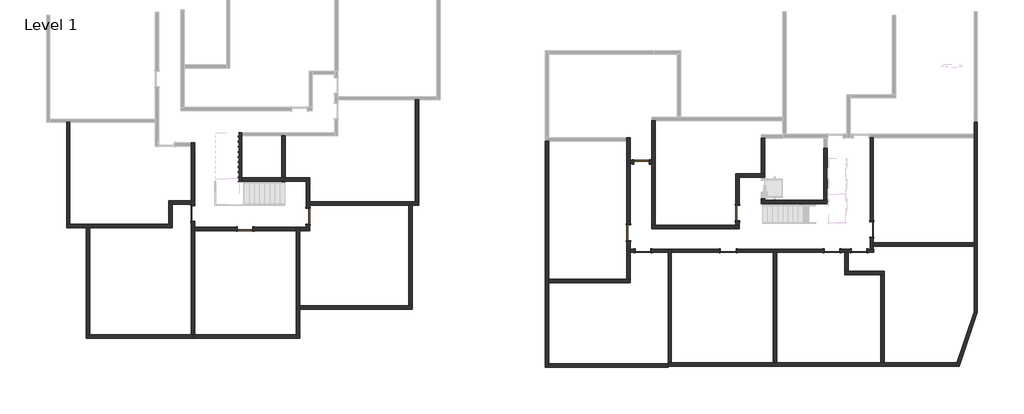
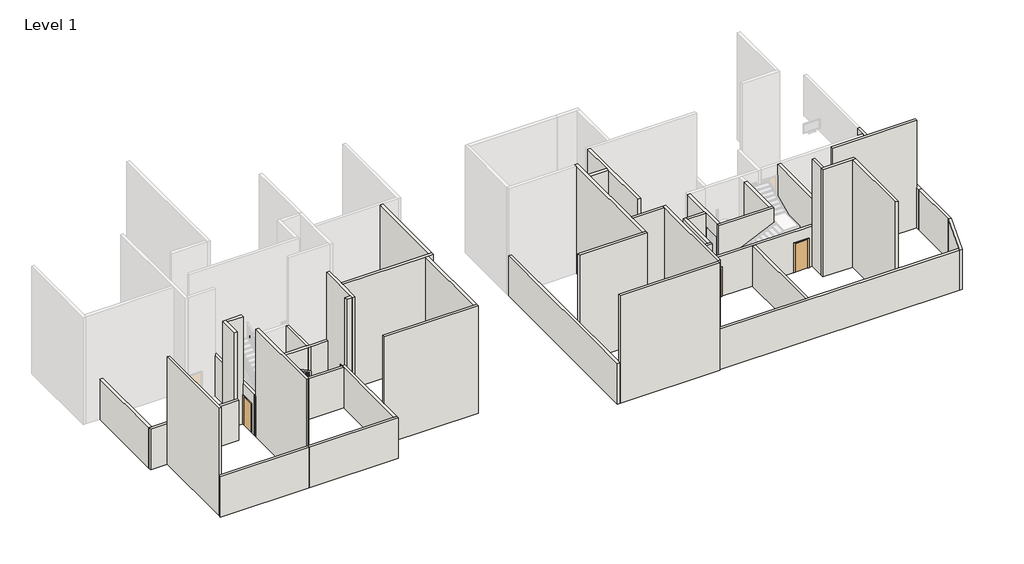
# One storey, part 1 of 3: 45 walls, 11 doors.
# Revit data of these elements (continued)
# Room at (24094.006, 1386.264) mm, phase "New Construction", upper level "Level 1", upper offset 243.84 cm, lower offset 0 cm (continued)
#   Name = "1"
# Room, not placed, phase "New Construction", upper offset 0 cm, lower offset 0 cm
#   Number = "81"
#   Name = "Room"
# Room, not placed, phase "New Construction", upper offset 0 cm, lower offset 0 cm
#   Number = "82"
#   Name = "Room"
# Room, not placed, phase "New Construction", upper offset 0 cm, lower offset 0 cm
#   Number = "83"
#   Name = "Room"
# Room, not placed, phase "New Construction", upper offset 0 cm, lower offset 0 cm
#   Number = "84"
#   Name = "5"
# Room, not placed, phase "New Construction", upper offset 0 cm, lower offset 0 cm
#   Number = "85"
#   Name = "Room"
# Room, not placed, phase "New Construction", upper offset 0 cm, lower offset 0 cm
#   Number = "18"
#   Name = "Room"
# Room, not placed, phase "New Construction", upper offset 0 cm, lower offset 0 cm
#   Number = "86"
#   Name = "Room"
# Room, not placed, phase "New Construction", upper offset 0 cm, lower offset 0 cm
#   Number = "137"
#   Name = "Room"
# Room at (15996.482, -9926.883) mm, phase "New Construction", upper level "Level 1", upper offset 243.84 cm, lower offset 0 cm
#   Number = "121"
#   Name = "5"
# Room at (9621.564, -11578.797) mm, phase "New Construction", upper level "Level 1", upper offset 243.84 cm, lower offset 0 cm
#   Number = "122"
#   Name = "6"
# Room at (20140.22, -1678.403) mm, phase "New Construction", upper level "Level 1", upper offset 243.84 cm, lower offset 0 cm
#   Number = ""
#   Name = "ASANSÖR"
# Room at (18694.214, -4908.781) mm, phase "New Construction", upper level "Level 1", upper offset 243.84 cm, lower offset 0 cm
#   Number = "49"
#   Name = "Room"
# Room, not placed, phase "New Construction", upper offset 0 cm, lower offset 0 cm
#   Number = "50"
#   Name = "Room"
# Room, not placed, phase "New Construction", upper offset 0 cm, lower offset 0 cm
#   Number = "51"
#   Name = "Room"
# Room, not placed, phase "New Construction", upper offset 0 cm, lower offset 0 cm
#   Number = "52"
#   Name = "Room"
# Room, not placed, phase "New Construction", upper offset 0 cm, lower offset 0 cm
#   Number = "53"
#   Name = "Room"
# Room, not placed, phase "New Construction", upper offset 0 cm, lower offset 0 cm
#   Number = "54"
#   Name = "Room"
# Room, not placed, phase "New Construction", upper offset 0 cm, lower offset 0 cm
#   Number = "55"
#   Name = "Room"
# Room, not placed, phase "New Construction", upper offset 0 cm, lower offset 0 cm
#   Number = "56"
#   Name = "Room"
# Room, not placed, phase "New Construction", upper offset 0 cm, lower offset 0 cm
#   Number = ""
#   Name = "Çamaşır- Kombi"
# Room, not placed, phase "New Construction", upper offset 0 cm, lower offset 0 cm
#   Number = "32"
#   Name = "Room"
# Room, not placed, phase "New Construction", upper offset 0 cm, lower offset 0 cm
#   Number = "33"
#   Name = "Room"
# Room at (7488.93, 2835.695) mm, phase "New Construction", upper level "Level 1", upper offset 243.84 cm, lower offset 0 cm
#   Number = "148"
#   Name = "8"
# Room at (7233.818, -6985.691) mm, phase "New Construction", upper level "Level 1", upper offset 243.84 cm, lower offset 0 cm
#   Number = "123"
#   Name = "7"
# Room, not placed, phase "New Construction", upper offset 0 cm, lower offset 0 cm
#   Number = "138"
#   Name = "Room"
# Room at (25542.506, -4072.569) mm, phase "New Construction", upper level "Level 1", upper offset 243.84 cm, lower offset 0 cm
#   Number = "87"
#   Name = "2"
# Room at (21725.305, -10013.945) mm, phase "New Construction", upper level "Level 1", upper offset 243.84 cm, lower offset 0 cm
#   Number = "88"
#   Name = "4"
# Area at (20046.111, 5871.007) mm, upper offset 243.84 cm, lower offset 0 cm
#   Number = "12"
#   Name = "Area"
# Room at (-4310.78, -978.519) mm, phase "New Construction", upper level "Level 1", upper offset 243.84 cm, lower offset 0 cm
#   Number = "149"
#   Name = "7"
# Room, not placed, phase "New Construction", upper offset 0 cm, lower offset 0 cm
#   Number = "57"
#   Name = "Room"
# Room, not placed, phase "New Construction", upper offset 0 cm, lower offset 0 cm
#   Number = ""
#   Name = "Room"
# Room, not placed, phase "New Construction", upper offset 0 cm, lower offset 0 cm
#   Number = "59"
#   Name = "Room"
# Room, not placed, phase "New Construction", upper offset 0 cm, lower offset 0 cm
#   Number = "60"
#   Name = "Room"
# Room, not placed, phase "New Construction", upper offset 0 cm, lower offset 0 cm
#   Number = "61"
#   Name = "Room"
# Room, not placed, phase "New Construction", upper offset 0 cm, lower offset 0 cm
#   Number = "62"
#   Name = "Room"
# Room, not placed, phase "New Construction", upper offset 0 cm, lower offset 0 cm
#   Number = "63"
#   Name = "Room"
# Area, not placed, upper offset 0 cm, lower offset 0 cm
#   Number = "5"
#   Name = "Dere Parsel Toplam Alan"
# Room, not placed, phase "New Construction", upper offset 0 cm, lower offset 0 cm
#   Number = "67"
#   Name = "Room"
# Room, not placed, phase "New Construction", upper offset 0 cm, lower offset 0 cm
#   Number = "68"
#   Name = "Room"
# Room at (-14817.024, 11588.139) mm, phase "New Construction", upper level "Level 1", upper offset 243.84 cm, lower offset 0 cm
#   Number = "139"
#   Name = "10"
# Room at (27717.749, -8269.379) mm, phase "New Construction", upper level "Level 1", upper offset 243.84 cm, lower offset 0 cm
#   Number = "90"
#   Name = "3"
# Area, not placed, upper offset 0 cm, lower offset 0 cm
#   Number = "6"
#   Name = "Area"
# Room, not placed, phase "New Construction", upper offset 0 cm, lower offset 0 cm
#   Number = "93"
#   Name = "6"
# Room, not placed, phase "New Construction", upper offset 0 cm, lower offset 0 cm
#   Number = "5"
#   Name = "Room"
# Room, not placed, phase "New Construction", upper offset 0 cm, lower offset 0 cm
#   Number = "6"
#   Name = "Room"
# Room, not placed, phase "New Construction", upper offset 0 cm, lower offset 0 cm
#   Number = "124"
#   Name = "Room"
# Room at (-20992.701, 5104.389) mm, phase "New Construction", upper level "Level 1", upper offset 243.84 cm, lower offset 0 cm
#   Number = "140"
#   Name = "2"
# Room at (-18388.177, -3094.154) mm, phase "New Construction", upper level "Level 1", upper offset 243.84 cm, lower offset 0 cm
#   Number = "141"
#   Name = "3"
# Room, not placed, phase "New Construction", upper offset 0 cm, lower offset 0 cm
#   Number = "34"
#   Name = "Room"
# Room, not placed, phase "New Construction", upper offset 0 cm, lower offset 0 cm
#   Number = "35"
#   Name = "Room"
# Room, not placed, phase "New Construction", upper offset 0 cm, lower offset 0 cm
#   Number = "9"
#   Name = "Room"
# Room, not placed, phase "New Construction", upper offset 0 cm, lower offset 0 cm
#   Number = "10"
#   Name = "Room"
# Room, not placed, phase "New Construction", upper offset 0 cm, lower offset 0 cm
#   Number = "125"
#   Name = "Room"
# Room, not placed, phase "New Construction", upper offset 0 cm, lower offset 0 cm
#   Number = "126"
#   Name = "Room"
# Room, not placed, phase "New Construction", upper offset 0 cm, lower offset 0 cm
#   Number = "127"
#   Name = "Room"
# Room, not placed, phase "New Construction", upper offset 0 cm, lower offset 0 cm
#   Number = "128"
#   Name = "Room"
# Room, not placed, phase "New Construction", upper offset 0 cm, lower offset 0 cm
#   Number = "129"
#   Name = "Room"
# Room, not placed, phase "New Construction", upper offset 0 cm, lower offset 0 cm
#   Number = "91"
#   Name = "Room"
# Room at (-21021.225, 8802.195) mm, phase "New Construction", upper level "Level 1", upper offset 243.84 cm, lower offset 0 cm
#   Number = "130"
#   Name = "1"
# Room at (-7083.952, -9470.79) mm, phase "New Construction", upper level "Level 1", upper offset 243.84 cm, lower offset 0 cm
#   Number = "131"
#   Name = "6"
# Room, not placed, phase "New Construction", upper offset 0 cm, lower offset 0 cm
#   Number = "132"
#   Name = "Room"
# Room, not placed, phase "New Construction", upper offset 0 cm, lower offset 0 cm
#   Number = "133"
#   Name = "Room"
# Room, not placed, phase "New Construction", upper offset 0 cm, lower offset 0 cm
#   Number = ""
#   Name = ""
# Room, not placed, phase "New Construction", upper offset 0 cm, lower offset 0 cm
#   Number = "70"
#   Name = "Room"
# Room, not placed, phase "New Construction", upper offset 0 cm, lower offset 0 cm
#   Number = "71"
#   Name = "Room"
# Room at (-18795.413, -7606.788) mm, phase "New Construction", upper level "Level 1", upper offset 243.84 cm, lower offset 0 cm
#   Number = "150"
#   Name = "4"
# Room at (43355.762, -8638.307) mm, phase "New Construction", upper level "Level 1", upper offset 243.84 cm, lower offset 0 cm
#   Number = "151"
#   Name = "Room"
# Room, not placed, phase "New Construction", upper offset 0 cm, lower offset 0 cm
#   Number = "92"
#   Name = "Room"
# Room, not placed, phase "New Construction", upper offset 0 cm, lower offset 0 cm
#   Number = ""
#   Name = ""
# Area, not placed, upper offset 0 cm, lower offset 0 cm
#   Number = "10"
#   Name = "Area"
# Area, not placed, upper offset 0 cm, lower offset 0 cm
#   Number = "11"
#   Name = "Area"
# Room, not placed, phase "New Construction", upper offset 0 cm, lower offset 0 cm
#   Number = ""
#   Name = ""
# Room, not placed, phase "New Construction", upper offset 0 cm, lower offset 0 cm
#   Number = "37"
#   Name = "Room"
# Room, not placed, phase "New Construction", upper offset 0 cm, lower offset 0 cm
#   Number = ""
#   Name = "Banyo"
# Room, not placed, phase "New Construction", upper offset 0 cm, lower offset 0 cm
#   Number = ""
#   Name = ""
# Room, not placed, phase "New Construction", upper offset 0 cm, lower offset 0 cm
#   Number = ""
#   Name = "Yatak Odası"
# Room, not placed, phase "New Construction", upper offset 0 cm, lower offset 0 cm
#   Number = "39"
#   Name = "Room"
# Room, not placed, phase "New Construction", upper offset 0 cm, lower offset 0 cm
#   Number = ""
#   Name = "Salon-Mutfak"
# Area, not placed, upper offset 0 cm, lower offset 0 cm
#   Number = "9"
#   Name = "Area"
# Room, not placed, phase "New Construction", upper offset 0 cm, lower offset 0 cm
#   Number = "134"
#   Name = "Room"
# Room, not placed, phase "New Construction", upper offset 0 cm, lower offset 0 cm
#   Number = "135"
#   Name = "Room"
# Room, not placed, phase "New Construction", upper offset 0 cm, lower offset 0 cm
#   Number = "40"
#   Name = "Room"
# Room, not placed, phase "New Construction", upper offset 0 cm, lower offset 0 cm
#   Number = "41"
#   Name = "Room"
# Room at (-12703.035, -7311.307) mm, phase "New Construction", upper level "Level 1", upper offset 243.84 cm, lower offset 0 cm
#   Number = "142"
#   Name = "5"
# Room, not placed, phase "New Construction", upper offset 0 cm, lower offset 0 cm
#   Number = "143"
#   Name = "Room"
# Room, not placed, phase "New Construction", upper offset 0 cm, lower offset 0 cm
#   Number = "144"
#   Name = "Room"
# Room at (-12608.918, 6644.855) mm, phase "New Construction", upper level "Level 1", upper offset 243.84 cm, lower offset 0 cm
#   Number = "145"
#   Name = "9"
# Room at (-5540.029, 3759.304) mm, phase "New Construction", upper level "Level 1", upper offset 243.84 cm, lower offset 0 cm
#   Number = "146"
#   Name = "8"
# Area, not placed, upper offset 0 cm, lower offset 0 cm
#   Number = "8"
#   Name = "Dere Parsel Toplam Alan"
# Room, not placed, phase "New Construction", upper offset 0 cm, lower offset 0 cm
#   Number = "108"
#   Name = "ASANSÖR"
# Room, not placed, phase "New Construction", upper offset 0 cm, lower offset 0 cm
#   Number = "89"
#   Name = "Room"
# Room, not placed, phase "New Construction", upper offset 0 cm, lower offset 0 cm
#   Number = "147"
#   Name = "Room"
# Room, not placed, phase "New Construction", upper offset 0 cm, lower offset 0 cm
#   Number = "19"
#   Name = "Room"
# Room, not placed, phase "New Construction", upper offset 0 cm, lower offset 0 cm
#   Number = ""
#   Name = ""
# Room, not placed, phase "New Construction", upper offset 0 cm, lower offset 0 cm
#   Number = "21"
#   Name = "Room"
# Room, not placed, phase "New Construction", upper offset 0 cm, lower offset 0 cm
#   Number = "22"
#   Name = "Room"
# Room, not placed, phase "New Construction", upper offset 0 cm, lower offset 0 cm
#   Number = "23"
#   Name = "Room"
# Room, not placed, phase "New Construction", upper offset 0 cm, lower offset 0 cm
#   Number = "24"
#   Name = "Room"
# Room, not placed, phase "New Construction", upper offset 0 cm, lower offset 0 cm
#   Number = "25"
#   Name = "Room"
# Room, not placed, phase "New Construction", upper offset 0 cm, lower offset 0 cm
#   Number = "64"
#   Name = "Room"
# Room, not placed, phase "New Construction", upper offset 0 cm, lower offset 0 cm
#   Number = "65"
#   Name = "Room"
# Room, not placed, phase "New Construction", upper offset 0 cm, lower offset 0 cm
#   Number = "66"
#   Name = "Room"
# Room, not placed, phase "New Construction", upper offset 0 cm, lower offset 0 cm
#   Number = ""
#   Name = ""
# Room, not placed, phase "New Construction", upper offset 0 cm, lower offset 0 cm
#   Number = "27"
#   Name = "Room"
# Room, not placed, phase "New Construction", upper offset 0 cm, lower offset 0 cm
#   Number = "42"
#   Name = "Room"
# Area, not placed, upper offset 0 cm, lower offset 0 cm
#   Number = "13"
#   Name = "Area"
# Area at (-15119.602, 13833.859) mm, upper offset 243.84 cm, lower offset 0 cm
#   Number = "14"
#   Name = "Area"
# Area, not placed, upper offset 0 cm, lower offset 0 cm
#   Number = "2"
#   Name = "Area"
# Room, not placed, phase "New Construction", upper offset 0 cm, lower offset 0 cm
#   Number = "43"
#   Name = "Room"
# Room, not placed, phase "New Construction", upper offset 0 cm, lower offset 0 cm
#   Number = ""
#   Name = ""
# Room, not placed, phase "New Construction", upper offset 0 cm, lower offset 0 cm
#   Number = "94"
#   Name = "Room"
# Room, not placed, phase "New Construction", upper offset 0 cm, lower offset 0 cm
#   Number = ""
#   Name = ""
# Room, not placed, phase "New Construction", upper offset 0 cm, lower offset 0 cm
#   Number = "136"
#   Name = "Room"
# Room, not placed, phase "New Construction", upper offset 0 cm, lower offset 0 cm
#   Number = "1"
#   Name = "Room"
# Area, not placed, upper offset 0 cm, lower offset 0 cm
#   Number = "3"
#   Name = "Area"
# Room, not placed, phase "New Construction", upper offset 0 cm, lower offset 0 cm
#   Number = "7"
#   Name = "Room"
# Room, not placed, phase "New Construction", upper offset 0 cm, lower offset 0 cm
#   Number = "8"
#   Name = "Room"
# Room, not placed, phase "New Construction", upper offset 0 cm, lower offset 0 cm
#   Number = "2"
#   Name = "Room"
# Room, not placed, phase "New Construction", upper offset 0 cm, lower offset 0 cm
#   Number = "46"
#   Name = "Room"
# Room, not placed, phase "New Construction", upper offset 0 cm, lower offset 0 cm
#   Number = "3"
#   Name = "Room"
# Room, not placed, phase "New Construction", upper offset 0 cm, lower offset 0 cm
#   Number = ""
#   Name = ""
# Room, not placed, phase "New Construction", upper offset 0 cm, lower offset 0 cm
#   Number = "4"
#   Name = "Room"
# Area, not placed, upper offset 0 cm, lower offset 0 cm
#   Number = "1"
#   Name = "Area"
# Room, not placed, phase "New Construction", upper offset 0 cm, lower offset 0 cm
#   Number = ""
#   Name = ""
# Room, not placed, phase "New Construction", upper offset 0 cm, lower offset 0 cm
#   Number = "29"
#   Name = "Room"
# Area, not placed, upper offset 0 cm, lower offset 0 cm
#   Number = "7"
#   Name = "Dere Parsel Toplam Alan"
# Room, not placed, phase "New Construction", upper offset 0 cm, lower offset 0 cm
#   Number = "95"
#   Name = "ASANSÖR"
# Room, not placed, phase "New Construction", upper offset 0 cm, lower offset 0 cm
#   Number = "96"
#   Name = "Room"
# Room, not placed, phase "New Construction", upper offset 0 cm, lower offset 0 cm
#   Number = "97"
#   Name = "7"
# Room, not placed, phase "New Construction", upper offset 0 cm, lower offset 0 cm
#   Number = "98"
#   Name = "8"
# Room, not placed, phase "New Construction", upper offset 0 cm, lower offset 0 cm
#   Number = "99"
#   Name = "9"
# Room, not placed, phase "New Construction", upper offset 0 cm, lower offset 0 cm
#   Number = "100"
#   Name = "1"
# Room, not placed, phase "New Construction", upper offset 0 cm, lower offset 0 cm
#   Number = "101"
#   Name = "5"
# Room, not placed, phase "New Construction", upper offset 0 cm, lower offset 0 cm
#   Number = "102"
#   Name = "2"
# Room, not placed, phase "New Construction", upper offset 0 cm, lower offset 0 cm
#   Number = "103"
#   Name = "4"
# Room, not placed, phase "New Construction", upper offset 0 cm, lower offset 0 cm
#   Number = "104"
#   Name = "3"
# Room, not placed, phase "New Construction", upper offset 0 cm, lower offset 0 cm
#   Number = "105"
#   Name = "6"
